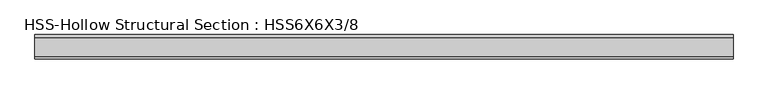
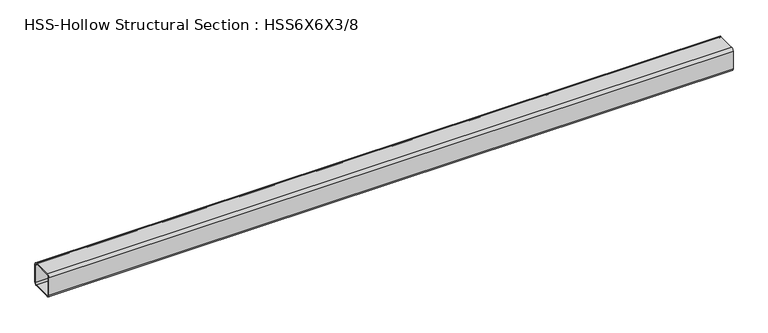
"""IFC4 building model written with IfcOpenShell, lengths in millimetres: member geometry, HSS-Hollow Structural Section : HSS6X6X3/8."""

import ifcopenshell
import ifcopenshell.guid

model = None  # the IFC model being written
_history = None  # IfcOwnerHistory: only IFC2X3 demands one
_inside = {}  # id of a spatial element -> (the spatial element, [elements in it])
_under = {}  # id of a project, library or spatial element -> (it, [spatial elements below it])
_declared = {}  # id of a project -> (the project, [libraries it declares])
_typed = {}  # id of a type object -> (the type object, [elements of that type])
_made_of = {}  # id of a material, layer set ... -> (it, [elements and type objects made of it])


def new_model(schema):
    """Start an empty IFC model of exactly this schema.

    Asked for "IFC4X3", IfcOpenShell would pick the latest addendum, in which some entities
    have other attributes; the version numbers below select the first issue.
    IFC2X3 requires an IfcOwnerHistory on every rooted entity: one is made here for all.
    """
    global model, _history
    if schema == "IFC4X3":
        model = ifcopenshell.file(schema_version=(4, 3, 0, 0))
    else:
        model = ifcopenshell.file(schema=schema)
    _inside.clear()
    _under.clear()
    _declared.clear()
    _typed.clear()
    _made_of.clear()
    _history = None
    if model.schema == "IFC2X3":
        org = make("IfcOrganization", Name="unknown")
        user = make(
            "IfcPersonAndOrganization",
            ThePerson=make("IfcPerson", FamilyName="unknown"),
            TheOrganization=org,
        )
        app = make(
            "IfcApplication",
            ApplicationDeveloper=org,
            Version="unknown",
            ApplicationFullName="unknown",
            ApplicationIdentifier="unknown",
        )
        _history = make(
            "IfcOwnerHistory",
            OwningUser=user,
            OwningApplication=app,
            ChangeAction="ADDED",
            CreationDate=0,
        )
    return model


def make(cls, **values):
    """One entity of the class cls with the attributes given. An attribute that is None is left unset."""
    return model.create_entity(
        cls, **{name: value for name, value in values.items() if value is not None}
    )


def rooted(cls, **values):
    """An entity with a GlobalId (a new one), such as an element, a storey or a relation."""
    return make(cls, GlobalId=ifcopenshell.guid.new(), OwnerHistory=_history, **values)


def si_unit(unit_type, name, prefix=None):
    """IfcSIUnit, for example si_unit("LENGTHUNIT", "METRE", prefix="MILLI")."""
    return make("IfcSIUnit", UnitType=unit_type, Prefix=prefix, Name=name)


def assignment(units):
    """IfcUnitAssignment: the units of a project."""
    return None if units is None else make("IfcUnitAssignment", Units=units)


def point(xyz):
    """IfcCartesianPoint."""
    return None if xyz is None else make("IfcCartesianPoint", Coordinates=xyz)


def direction(xyz):
    """IfcDirection."""
    return None if xyz is None else make("IfcDirection", DirectionRatios=xyz)


def frame(location, z_axis=None, x_axis=None):
    """IfcAxis2Placement3D, a coordinate frame: its origin and axes. An axis left out is left unset."""
    return make(
        "IfcAxis2Placement3D",
        Location=point(location),
        Axis=direction(z_axis),
        RefDirection=direction(x_axis),
    )


def frame_2d(location, x_axis=None):
    """IfcAxis2Placement2D, a coordinate frame in the plane: its origin and x axis."""
    return make(
        "IfcAxis2Placement2D", Location=point(location), RefDirection=direction(x_axis)
    )


def origin():
    """The frame at (0, 0, 0) with its axes left unset."""
    return frame((0.0, 0.0, 0.0))


def place(relative_to, where):
    """IfcLocalPlacement: puts the frame where relative to a parent placement (None: the world)."""
    return make(
        "IfcLocalPlacement", PlacementRelTo=relative_to, RelativePlacement=where
    )


def context(
    kind, dimensions, precision=None, world=None, true_north=None, identifier=None
):
    """IfcGeometricRepresentationContext, for example the 3D "Model" context."""
    return make(
        "IfcGeometricRepresentationContext",
        ContextIdentifier=identifier,
        ContextType=kind,
        CoordinateSpaceDimension=dimensions,
        Precision=precision,
        WorldCoordinateSystem=world,
        TrueNorth=true_north,
    )


def project(units=None, contexts=None):
    """IfcProject with its units and contexts."""
    return rooted(
        "IfcProject",
        Name="project",
        RepresentationContexts=contexts,
        UnitsInContext=assignment(units),
    )


def spatial(cls, under=None, at=None, **own):
    """A site, building, storey or space (cls), placed at a placement, below another one or the project."""
    s = rooted(cls, ObjectPlacement=at, **own)
    if under is not None:
        _under.setdefault(under.id(), (under, []))[1].append(s)
    return s


def polyline(points):
    """IfcPolyline through the points."""
    return make("IfcPolyline", Points=[point(p) for p in points])


def circle_curve(where, radius):
    """IfcCircle in the frame where."""
    return make("IfcCircle", Position=where, Radius=radius)


def trimmed(basis, trim1, trim2, sense, master):
    """IfcTrimmedCurve: the piece of a basis curve between two trims."""
    return make(
        "IfcTrimmedCurve",
        BasisCurve=basis,
        Trim1=trim1,
        Trim2=trim2,
        SenseAgreement=sense,
        MasterRepresentation=master,
    )


def segment(curve, same_sense, transition):
    """IfcCompositeCurveSegment."""
    return make(
        "IfcCompositeCurveSegment",
        Transition=transition,
        SameSense=same_sense,
        ParentCurve=curve,
    )


def composite_curve(segments, self_intersect=None):
    """IfcCompositeCurve: segments joined end to end."""
    return make("IfcCompositeCurve", Segments=segments, SelfIntersect=self_intersect)


def outline(outer, holes=None, kind="AREA"):
    """IfcArbitraryClosedProfileDef: a profile drawn as a closed curve; with holes, ...WithVoids."""
    if holes is None:
        return make("IfcArbitraryClosedProfileDef", ProfileType=kind, OuterCurve=outer)
    return make(
        "IfcArbitraryProfileDefWithVoids",
        ProfileType=kind,
        OuterCurve=outer,
        InnerCurves=holes,
    )


def extrude(swept, where, along, depth):
    """IfcExtrudedAreaSolid: the profile swept, set in the frame where, extruded along a direction by depth."""
    return make(
        "IfcExtrudedAreaSolid",
        SweptArea=swept,
        Position=where,
        ExtrudedDirection=direction(along),
        Depth=depth,
    )


def shape(context_of_items, identifier, shape_type, items):
    """IfcShapeRepresentation: the items that make up one representation, for example the "Body"."""
    return make(
        "IfcShapeRepresentation",
        ContextOfItems=context_of_items,
        RepresentationIdentifier=identifier,
        RepresentationType=shape_type,
        Items=items,
    )


def source(mapping_origin, context_of_items, identifier, shape_type, items):
    """IfcRepresentationMap: a shape defined once, which mapped items show again and again."""
    return make(
        "IfcRepresentationMap",
        MappingOrigin=mapping_origin,
        MappedRepresentation=shape(context_of_items, identifier, shape_type, items),
    )


def transform(
    local_origin,
    x_axis=None,
    y_axis=None,
    z_axis=None,
    scale=None,
    scale2=None,
    scale3=None,
    uniform=True,
):
    """IfcCartesianTransformationOperator3D, or its non-uniform kind. x_axis, y_axis, z_axis: its Axis1, 2, 3."""
    if uniform:
        return make(
            "IfcCartesianTransformationOperator3D",
            Axis1=direction(x_axis),
            Axis2=direction(y_axis),
            LocalOrigin=point(local_origin),
            Scale=scale,
            Axis3=direction(z_axis),
        )
    return make(
        "IfcCartesianTransformationOperator3DnonUniform",
        Axis1=direction(x_axis),
        Axis2=direction(y_axis),
        LocalOrigin=point(local_origin),
        Scale=scale,
        Axis3=direction(z_axis),
        Scale2=scale2,
        Scale3=scale3,
    )


def mapped(mapping_source, mapping_target):
    """IfcMappedItem: shows the shape of a source again, moved by a transform."""
    return make(
        "IfcMappedItem", MappingSource=mapping_source, MappingTarget=mapping_target
    )


def made_of(thing, what):
    """Note that an element or type object is made of a material, layer set ...; save() writes the relation."""
    if what is not None:
        _made_of.setdefault(what.id(), (what, []))[1].append(thing)
    return thing


def element(
    cls,
    number,
    at=None,
    inside=None,
    cuts=None,
    type_object=None,
    material=None,
    context=None,
    identifier="Body",
    shape_type=None,
    held_by="IfcProductDefinitionShape",
    body=None,
    shapes=None,
    **own,
):
    """One element of the class cls, such as IfcWall. Its Tag is "e" and its number.

    at: its placement. inside: the storey or other place that contains it. cuts: it is an
    opening in that element (IfcRelVoidsElement). A single representation is given by context,
    identifier, shape_type and body (its items); several are given by shapes. held_by: the class
    of the entity that holds the representations. save() writes the other relations.
    """
    e = rooted(cls, Tag="e%d" % number, ObjectPlacement=at, **own)
    if body is not None:
        shapes = [shape(context, identifier, shape_type, body)]
    if shapes is not None:
        e.Representation = make(held_by, Representations=shapes)
    if inside is not None:
        _inside.setdefault(inside.id(), (inside, []))[1].append(e)
    if cuts is not None:
        rooted(
            "IfcRelVoidsElement", RelatingBuildingElement=cuts, RelatedOpeningElement=e
        )
    if type_object is not None:
        _typed.setdefault(type_object.id(), (type_object, []))[1].append(e)
    return made_of(e, material)


def aggregate(whole, parts):
    """IfcRelAggregates: a whole, such as a stair, and the parts it consists of."""
    return rooted("IfcRelAggregates", RelatingObject=whole, RelatedObjects=parts)


def save(model, path):
    """Write the relations noted so far, then the file.

    IfcRelAggregates (storeys below a building ...), IfcRelContainedInSpatialStructure (elements
    in a storey), IfcRelDefinesByType, IfcRelAssociatesMaterial and IfcRelDeclares: one each for
    every whole, place, type object, material and project.
    """
    for whole, parts in _under.values():
        aggregate(whole, parts)
    for where, things in _inside.values():
        rooted(
            "IfcRelContainedInSpatialStructure",
            RelatedElements=things,
            RelatingStructure=where,
        )
    for kind, things in _typed.values():
        rooted("IfcRelDefinesByType", RelatedObjects=things, RelatingType=kind)
    for what, things in _made_of.values():
        rooted("IfcRelAssociatesMaterial", RelatedObjects=things, RelatingMaterial=what)
    for by, libraries in _declared.values():
        rooted("IfcRelDeclares", RelatingContext=by, RelatedDefinitions=libraries)
    model.write(path)


def hss_hollow_structural_section_hss6x6x3_8_c14c5591(model_context):
    return source(origin(), model_context, "Body", "SweptSolid", [
        extrude(outline(composite_curve([segment(polyline([(76.2, 58.4708), (76.2, -58.4708)]), True, "CONTINUOUS"), segment(trimmed(circle_curve(frame_2d((58.4708, -58.4708)), 17.7292), [point((76.2, -58.4708))], [point((58.4708, -76.2))], False, "CARTESIAN"), True, "CONTINUOUS"), segment(polyline([(58.4708, -76.2), (-58.4708, -76.2)]), True, "CONTINUOUS"), segment(trimmed(circle_curve(frame_2d((-58.4708, -58.4708)), 17.7292), [point((-58.4708, -76.2))], [point((-76.2, -58.4708))], False, "CARTESIAN"), True, "CONTINUOUS"), segment(polyline([(-76.2, -58.4708), (-76.2, 58.4708)]), True, "CONTINUOUS"), segment(trimmed(circle_curve(frame_2d((-58.4708, 58.4708)), 17.7292), [point((-76.2, 58.4708))], [point((-58.4708, 76.2))], False, "CARTESIAN"), True, "CONTINUOUS"), segment(polyline([(-58.4708, 76.2), (58.4708, 76.2)]), True, "CONTINUOUS"), segment(trimmed(circle_curve(frame_2d((58.4708, 58.4708)), 17.7292), [point((58.4708, 76.2))], [point((76.2, 58.4708))], False, "CARTESIAN"), True, "CONTINUOUS")], self_intersect=False), holes=[composite_curve([segment(trimmed(circle_curve(frame_2d((-58.4708, 58.4708)), 8.8646), [point((-58.4708, 67.3354))], [point((-67.3354, 58.4708))], True, "CARTESIAN"), True, "CONTINUOUS"), segment(polyline([(-67.3354, 58.4708), (-67.3354, -58.4708)]), True, "CONTINUOUS"), segment(trimmed(circle_curve(frame_2d((-58.4708, -58.4708)), 8.8646), [point((-67.3354, -58.4708))], [point((-58.4708, -67.3354))], True, "CARTESIAN"), True, "CONTINUOUS"), segment(polyline([(-58.4708, -67.3354), (58.4708, -67.3354)]), True, "CONTINUOUS"), segment(trimmed(circle_curve(frame_2d((58.4708, -58.4708)), 8.8646), [point((58.4708, -67.3354))], [point((67.3354, -58.4708))], True, "CARTESIAN"), True, "CONTINUOUS"), segment(polyline([(67.3354, -58.4708), (67.3354, 58.4708)]), True, "CONTINUOUS"), segment(trimmed(circle_curve(frame_2d((58.4708, 58.4708)), 8.8646), [point((67.3354, 58.4708))], [point((58.4708, 67.3354))], True, "CARTESIAN"), True, "CONTINUOUS"), segment(polyline([(58.4708, 67.3354), (-58.4708, 67.3354)]), True, "CONTINUOUS")], self_intersect=False)]), frame((-2169.5251939, 0.0, 0.0), z_axis=(1.0, 0.0, 0.0), x_axis=(0.0, 1.0, 0.0)), (0.0, 0.0, 1.0), 4339.0503878),
    ])


if __name__ == "__main__":
    model = new_model("IFC4")
    model_context = context("Model", 3, world=origin())
    ifc_project = project(units=[si_unit("LENGTHUNIT", "METRE", prefix="MILLI")], contexts=[model_context])
    site = spatial("IfcSite", under=ifc_project)
    building = spatial("IfcBuilding", under=site)
    placement = place(None, origin())
    hss_hollow_structural_section_hss6x6x3_8_shape = hss_hollow_structural_section_hss6x6x3_8_c14c5591(model_context)
    element("IfcMember", 1, ObjectType="HSS-Hollow Structural Section : HSS6X6X3/8", at=placement, inside=building, context=model_context, shape_type="MappedRepresentation", body=[
        mapped(hss_hollow_structural_section_hss6x6x3_8_shape, transform((0.0, 0.0, 0.0), x_axis=(1.0, 0.0, 0.0), y_axis=(0.0, 1.0, 0.0), z_axis=(0.0, 0.0, 1.0))),
    ])
    save(model, "model.ifc")

# Revit data of these elements
# Type "HSS-Hollow Structural Section : HSS6X6X3/8"
#   Assembly Code = "B10"
#   Shape = "Square"
#   W = 27.4
#   Ht = 0' - 6"
#   Length [instance default] = 5' - 0"
#   b = 0' - 6"
#   kr = 0' - 0.698"
#   t = 0' - 0.349"
#   A = 0.0526389 SF
#   Structural Material [instance default] = Steel ASTM A500, Grade B, Rectangular and Square
# Element 1 (IfcMember, "HSS-Hollow Structural Section : HSS6X6X3/8")
#   Materials on its faces: "Steel ASTM A500, Grade B, Rectangular and Square"
# Materials
#   "Steel ASTM A500, Grade B, Rectangular and Square": class "Metal", colour RGB 199 199 199, transparency 0, Description = "Carbon steel", Cost = 0
